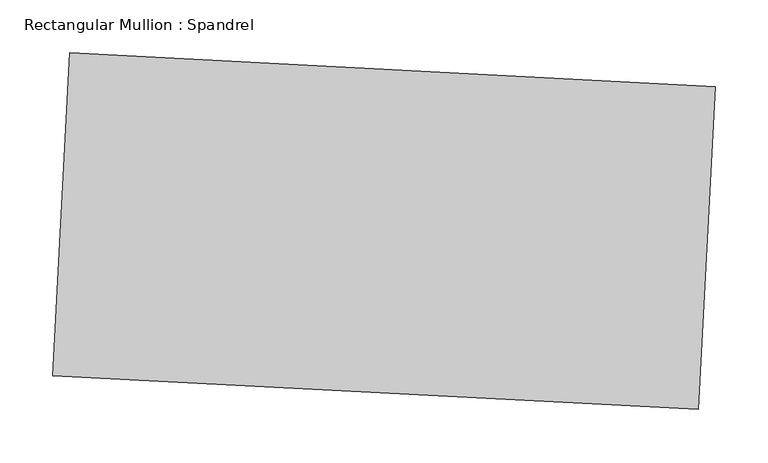
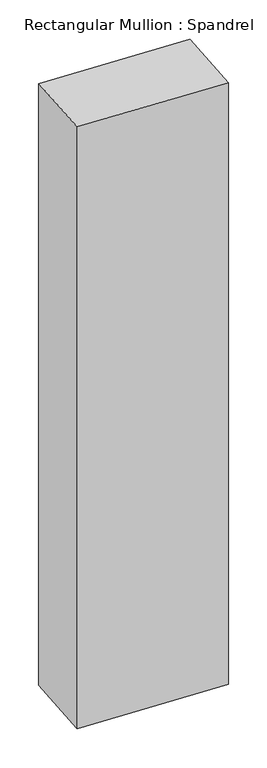
"""IFC4 building model written with IfcOpenShell, lengths in millimetres: member geometry, Rectangular Mullion : Spandrel."""

import ifcopenshell
import ifcopenshell.guid

model = None  # the IFC model being written
_history = None  # IfcOwnerHistory: only IFC2X3 demands one
_inside = {}  # id of a spatial element -> (the spatial element, [elements in it])
_under = {}  # id of a project, library or spatial element -> (it, [spatial elements below it])
_declared = {}  # id of a project -> (the project, [libraries it declares])
_typed = {}  # id of a type object -> (the type object, [elements of that type])
_made_of = {}  # id of a material, layer set ... -> (it, [elements and type objects made of it])


def new_model(schema):
    """Start an empty IFC model of exactly this schema.

    Asked for "IFC4X3", IfcOpenShell would pick the latest addendum, in which some entities
    have other attributes; the version numbers below select the first issue.
    IFC2X3 requires an IfcOwnerHistory on every rooted entity: one is made here for all.
    """
    global model, _history
    if schema == "IFC4X3":
        model = ifcopenshell.file(schema_version=(4, 3, 0, 0))
    else:
        model = ifcopenshell.file(schema=schema)
    _inside.clear()
    _under.clear()
    _declared.clear()
    _typed.clear()
    _made_of.clear()
    _history = None
    if model.schema == "IFC2X3":
        org = make("IfcOrganization", Name="unknown")
        user = make(
            "IfcPersonAndOrganization",
            ThePerson=make("IfcPerson", FamilyName="unknown"),
            TheOrganization=org,
        )
        app = make(
            "IfcApplication",
            ApplicationDeveloper=org,
            Version="unknown",
            ApplicationFullName="unknown",
            ApplicationIdentifier="unknown",
        )
        _history = make(
            "IfcOwnerHistory",
            OwningUser=user,
            OwningApplication=app,
            ChangeAction="ADDED",
            CreationDate=0,
        )
    return model


def make(cls, **values):
    """One entity of the class cls with the attributes given. An attribute that is None is left unset."""
    return model.create_entity(
        cls, **{name: value for name, value in values.items() if value is not None}
    )


def rooted(cls, **values):
    """An entity with a GlobalId (a new one), such as an element, a storey or a relation."""
    return make(cls, GlobalId=ifcopenshell.guid.new(), OwnerHistory=_history, **values)


def si_unit(unit_type, name, prefix=None):
    """IfcSIUnit, for example si_unit("LENGTHUNIT", "METRE", prefix="MILLI")."""
    return make("IfcSIUnit", UnitType=unit_type, Prefix=prefix, Name=name)


def assignment(units):
    """IfcUnitAssignment: the units of a project."""
    return None if units is None else make("IfcUnitAssignment", Units=units)


def point(xyz):
    """IfcCartesianPoint."""
    return None if xyz is None else make("IfcCartesianPoint", Coordinates=xyz)


def direction(xyz):
    """IfcDirection."""
    return None if xyz is None else make("IfcDirection", DirectionRatios=xyz)


def frame(location, z_axis=None, x_axis=None):
    """IfcAxis2Placement3D, a coordinate frame: its origin and axes. An axis left out is left unset."""
    return make(
        "IfcAxis2Placement3D",
        Location=point(location),
        Axis=direction(z_axis),
        RefDirection=direction(x_axis),
    )


def origin():
    """The frame at (0, 0, 0) with its axes left unset."""
    return frame((0.0, 0.0, 0.0))


def place(relative_to, where):
    """IfcLocalPlacement: puts the frame where relative to a parent placement (None: the world)."""
    return make(
        "IfcLocalPlacement", PlacementRelTo=relative_to, RelativePlacement=where
    )


def context(
    kind, dimensions, precision=None, world=None, true_north=None, identifier=None
):
    """IfcGeometricRepresentationContext, for example the 3D "Model" context."""
    return make(
        "IfcGeometricRepresentationContext",
        ContextIdentifier=identifier,
        ContextType=kind,
        CoordinateSpaceDimension=dimensions,
        Precision=precision,
        WorldCoordinateSystem=world,
        TrueNorth=true_north,
    )


def project(units=None, contexts=None):
    """IfcProject with its units and contexts."""
    return rooted(
        "IfcProject",
        Name="project",
        RepresentationContexts=contexts,
        UnitsInContext=assignment(units),
    )


def spatial(cls, under=None, at=None, **own):
    """A site, building, storey or space (cls), placed at a placement, below another one or the project."""
    s = rooted(cls, ObjectPlacement=at, **own)
    if under is not None:
        _under.setdefault(under.id(), (under, []))[1].append(s)
    return s


def polyline(points):
    """IfcPolyline through the points."""
    return make("IfcPolyline", Points=[point(p) for p in points])


def outline(outer, holes=None, kind="AREA"):
    """IfcArbitraryClosedProfileDef: a profile drawn as a closed curve; with holes, ...WithVoids."""
    if holes is None:
        return make("IfcArbitraryClosedProfileDef", ProfileType=kind, OuterCurve=outer)
    return make(
        "IfcArbitraryProfileDefWithVoids",
        ProfileType=kind,
        OuterCurve=outer,
        InnerCurves=holes,
    )


def extrude(swept, where, along, depth):
    """IfcExtrudedAreaSolid: the profile swept, set in the frame where, extruded along a direction by depth."""
    return make(
        "IfcExtrudedAreaSolid",
        SweptArea=swept,
        Position=where,
        ExtrudedDirection=direction(along),
        Depth=depth,
    )


def shape(context_of_items, identifier, shape_type, items):
    """IfcShapeRepresentation: the items that make up one representation, for example the "Body"."""
    return make(
        "IfcShapeRepresentation",
        ContextOfItems=context_of_items,
        RepresentationIdentifier=identifier,
        RepresentationType=shape_type,
        Items=items,
    )


def source(mapping_origin, context_of_items, identifier, shape_type, items):
    """IfcRepresentationMap: a shape defined once, which mapped items show again and again."""
    return make(
        "IfcRepresentationMap",
        MappingOrigin=mapping_origin,
        MappedRepresentation=shape(context_of_items, identifier, shape_type, items),
    )


def transform(
    local_origin,
    x_axis=None,
    y_axis=None,
    z_axis=None,
    scale=None,
    scale2=None,
    scale3=None,
    uniform=True,
):
    """IfcCartesianTransformationOperator3D, or its non-uniform kind. x_axis, y_axis, z_axis: its Axis1, 2, 3."""
    if uniform:
        return make(
            "IfcCartesianTransformationOperator3D",
            Axis1=direction(x_axis),
            Axis2=direction(y_axis),
            LocalOrigin=point(local_origin),
            Scale=scale,
            Axis3=direction(z_axis),
        )
    return make(
        "IfcCartesianTransformationOperator3DnonUniform",
        Axis1=direction(x_axis),
        Axis2=direction(y_axis),
        LocalOrigin=point(local_origin),
        Scale=scale,
        Axis3=direction(z_axis),
        Scale2=scale2,
        Scale3=scale3,
    )


def mapped(mapping_source, mapping_target):
    """IfcMappedItem: shows the shape of a source again, moved by a transform."""
    return make(
        "IfcMappedItem", MappingSource=mapping_source, MappingTarget=mapping_target
    )


def made_of(thing, what):
    """Note that an element or type object is made of a material, layer set ...; save() writes the relation."""
    if what is not None:
        _made_of.setdefault(what.id(), (what, []))[1].append(thing)
    return thing


def element(
    cls,
    number,
    at=None,
    inside=None,
    cuts=None,
    type_object=None,
    material=None,
    context=None,
    identifier="Body",
    shape_type=None,
    held_by="IfcProductDefinitionShape",
    body=None,
    shapes=None,
    **own,
):
    """One element of the class cls, such as IfcWall. Its Tag is "e" and its number.

    at: its placement. inside: the storey or other place that contains it. cuts: it is an
    opening in that element (IfcRelVoidsElement). A single representation is given by context,
    identifier, shape_type and body (its items); several are given by shapes. held_by: the class
    of the entity that holds the representations. save() writes the other relations.
    """
    e = rooted(cls, Tag="e%d" % number, ObjectPlacement=at, **own)
    if body is not None:
        shapes = [shape(context, identifier, shape_type, body)]
    if shapes is not None:
        e.Representation = make(held_by, Representations=shapes)
    if inside is not None:
        _inside.setdefault(inside.id(), (inside, []))[1].append(e)
    if cuts is not None:
        rooted(
            "IfcRelVoidsElement", RelatingBuildingElement=cuts, RelatedOpeningElement=e
        )
    if type_object is not None:
        _typed.setdefault(type_object.id(), (type_object, []))[1].append(e)
    return made_of(e, material)


def aggregate(whole, parts):
    """IfcRelAggregates: a whole, such as a stair, and the parts it consists of."""
    return rooted("IfcRelAggregates", RelatingObject=whole, RelatedObjects=parts)


def save(model, path):
    """Write the relations noted so far, then the file.

    IfcRelAggregates (storeys below a building ...), IfcRelContainedInSpatialStructure (elements
    in a storey), IfcRelDefinesByType, IfcRelAssociatesMaterial and IfcRelDeclares: one each for
    every whole, place, type object, material and project.
    """
    for whole, parts in _under.values():
        aggregate(whole, parts)
    for where, things in _inside.values():
        rooted(
            "IfcRelContainedInSpatialStructure",
            RelatedElements=things,
            RelatingStructure=where,
        )
    for kind, things in _typed.values():
        rooted("IfcRelDefinesByType", RelatedObjects=things, RelatingType=kind)
    for what, things in _made_of.values():
        rooted("IfcRelAssociatesMaterial", RelatedObjects=things, RelatingMaterial=what)
    for by, libraries in _declared.values():
        rooted("IfcRelDeclares", RelatingContext=by, RelatedDefinitions=libraries)
    model.write(path)


def rectangular_mullion_spandrel_46039ac9(model_context):
    return source(origin(), model_context, "Body", "SweptSolid", [
        extrude(outline(polyline([(312.3582819, 136.2391416), (296.4062825, -168.1431406), (-312.3582819, -136.2391416), (-296.4062825, 168.1431406), (312.3582819, 136.2391416)])), frame((0.0, 0.0, -2637.6144376), z_axis=(0.0, 0.0, 1.0), x_axis=(1.0, 0.0, 0.0)), (0.0, 0.0, 1.0), 2637.6144376),
    ])


if __name__ == "__main__":
    model = new_model("IFC4")
    model_context = context("Model", 3, world=origin())
    ifc_project = project(units=[si_unit("LENGTHUNIT", "METRE", prefix="MILLI")], contexts=[model_context])
    site = spatial("IfcSite", under=ifc_project)
    building = spatial("IfcBuilding", under=site)
    placement = place(None, origin())
    rectangular_mullion_spandrel_shape = rectangular_mullion_spandrel_46039ac9(model_context)
    element("IfcMember", 1, ObjectType="Rectangular Mullion : Spandrel", at=placement, inside=building, context=model_context, shape_type="MappedRepresentation", body=[
        mapped(rectangular_mullion_spandrel_shape, transform((0.0, 0.0, 0.0), x_axis=(1.0, 0.0, 0.0), y_axis=(0.0, 1.0, 0.0), z_axis=(0.0, 0.0, 1.0))),
    ])
    save(model, "model.ifc")

# Revit data of these elements
# Type "Rectangular Mullion : Spandrel"
#   built-in parameter 1007304 = 1 (stored number, unit not read)
#   built-in parameter 1007301 = 1 (stored number, unit not read)
#   built-in parameter 1007300 = 1 (stored number, unit not read)
# Element 1 (IfcMember, "Rectangular Mullion : Spandrel")
#   Materials on its faces: "Aluminum"
# Materials
#   "Aluminum": class "Metal", colour RGB 247 247 247, transparency 0, Description = "Aluminum 6061", Cost = 0
